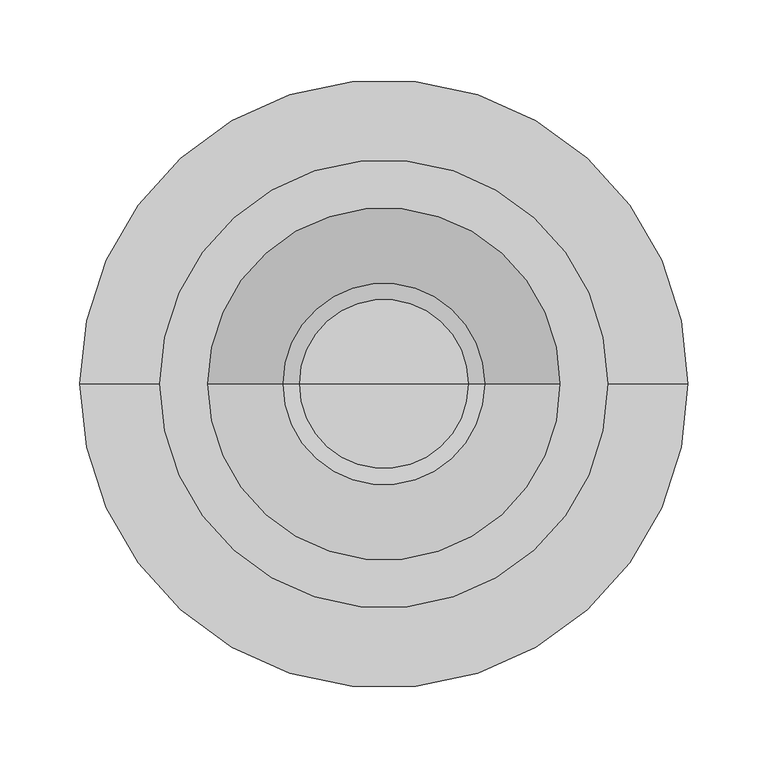
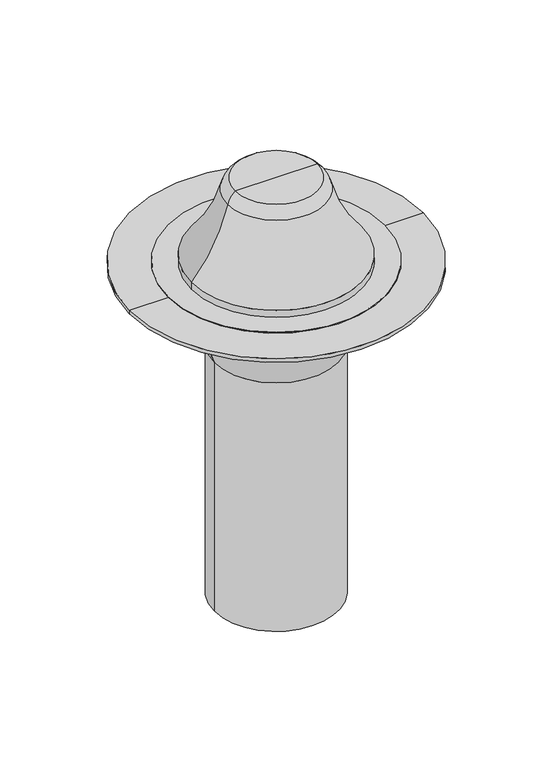
"""IFC4 building model written with IfcOpenShell, lengths in millimetres: proxy geometry, TN_Воронка с обжимным фланцем : Воронка с обжимным закручивающемся фланцем с обогревом Ø160х450мм."""

from ifc_helpers import new_model, si_unit, point, frame, origin, origin_with_axes, origin_2d, place, context, project, spatial, polyline, circle_curve, ellipse_curve, trimmed, segment, composite_curve, outline, extrude, source, transform, mapped, element, save
from ifc_brep_helpers import plane_surface, cylinder_surface, revolved_surface, advanced_brep


def specialty_equipment_53f7e9e1(model_context):
    return source(origin(), model_context, "Body", "SolidModel", [
        advanced_brep(
        [(110.0556416, 0.0, 0.0), (-110.0556416, 0.0, 0.0), (-110.0556416, 0.0, 10.0), (110.0556416, 0.0, 10.0), (0.0, 0.0, 0.0), (52.7728393, 0.0, 115.0), (-52.7728393, 0.0, 115.0), (0.0, 0.0, 115.0), (62.9807579, 0.0, 100.6532382), (-62.9807579, 0.0, 100.6532382)],
        [
            (0, 1, circle_curve(frame((0.0, 0.0, 0.0), z_axis=(0.0, 0.0, 1.0), x_axis=(-1.0, 0.0, 0.0)), 110.0556416)),
            (1, 2),
            (2, 3, circle_curve(frame((0.0, 0.0, 10.0), z_axis=(0.0, 0.0, -1.0), x_axis=(-1.0, 0.0, 0.0)), 110.0556416)),
            (3, 0),
            (1, 0, circle_curve(frame((0.0, 0.0, 0.0), z_axis=(0.0, 0.0, 1.0), x_axis=(-1.0, 0.0, 0.0)), 110.0556416)),
            (3, 2, circle_curve(frame((0.0, 0.0, 10.0), z_axis=(0.0, 0.0, -1.0), x_axis=(-1.0, 0.0, 0.0)), 110.0556416)),
            (4, 1),
            (0, 4),
            (5, 6, circle_curve(frame((0.0, 0.0, 115.0), z_axis=(0.0, 0.0, 1.0), x_axis=(-1.0, 0.0, 0.0)), 52.7728393)),
            (6, 7),
            (7, 5),
            (6, 5, circle_curve(frame((0.0, 0.0, 115.0), z_axis=(0.0, 0.0, 1.0), x_axis=(-1.0, 0.0, 0.0)), 52.7728393)),
            (8, 9, circle_curve(frame((0.0, 0.0, 100.6532382), z_axis=(0.0, 0.0, 1.0), x_axis=(-1.0, 0.0, 0.0)), 62.9807579)),
            (9, 6, circle_curve(frame((-39.8885443, 0.0, 95.0277285), z_axis=(0.0, 1.0, 0.0), x_axis=(1.0, 0.0, 0.0)), 23.7675553)),
            (5, 8, circle_curve(frame((39.8885443, 0.0, 95.0277285), z_axis=(0.0, 1.0, 0.0), x_axis=(-1.0, 0.0, 0.0)), 23.7675553)),
            (9, 8, circle_curve(frame((0.0, 0.0, 100.6532382), z_axis=(0.0, 0.0, 1.0), x_axis=(-1.0, 0.0, 0.0)), 62.9807579)),
            (2, 9, circle_curve(frame((-271.7387744, 0.0, 151.5089197), z_axis=(0.0, -1.0, 0.0), x_axis=(1.0, 0.0, 0.0)), 214.8632351)),
            (8, 3, circle_curve(frame((271.7387744, 0.0, 151.5089197), z_axis=(0.0, -1.0, 0.0), x_axis=(-1.0, 0.0, 0.0)), 214.8632351)),
        ],
        [
            cylinder_surface(frame((0.0, 0.0, 0.0), z_axis=(0.0, 0.0, -1.0), x_axis=(-1.0, 0.0, 0.0)), 110.0556416),
            plane_surface(frame((0.0, 0.0, 0.0), z_axis=(0.0, 0.0, -1.0), x_axis=(-1.0, 0.0, 0.0))),
            plane_surface(frame((0.0, 0.0, 115.0), z_axis=(0.0, 0.0, 1.0), x_axis=(-1.0, 0.0, 0.0))),
            revolved_surface(trimmed(ellipse_curve(frame((-39.8885443, 0.0, 95.0277285), z_axis=(0.0, -1.0, 0.0), x_axis=(1.0, 0.0, 0.0)), 23.7675553, 23.7675553), [point((-52.7728393, 0.0, 115.0))], [point((-62.9807579, 0.0, 100.6532382))], True, "CARTESIAN"), (0.0, 0.0, 0.0), (0.0, 0.0, -1.0)),
            revolved_surface(trimmed(ellipse_curve(frame((-271.7387744, 0.0, 151.5089197), z_axis=(0.0, 1.0, 0.0), x_axis=(1.0, 0.0, 0.0)), 214.8632351, 214.8632351), [point((-62.9807579, 0.0, 100.6532382))], [point((-110.0556416, 0.0, 10.0))], True, "CARTESIAN"), (0.0, 0.0, 0.0), (0.0, 0.0, -1.0)),
        ],
        [
            (0, [[1, 2, 3, 4]]),
            (0, [[5, -4, 6, -2]]),
            (1, [[7, -1, 8]]),
            (1, [[-8, -5, -7]]),
            (2, [[9, 10, 11]]),
            (2, [[12, -11, -10]]),
            (3, [[13, 14, -9, 15]]),
            (3, [[16, -15, -12, -14]]),
            (4, [[-3, 17, -13, 18]]),
            (4, [[-6, -18, -16, -17]]),
        ],
    ),
        extrude(outline(composite_curve([segment(trimmed(circle_curve(origin_2d(), 140.0), [point((-140.0, 0.0))], [point((140.0, 0.0))], False, "CARTESIAN"), True, "CONTINUOUS"), segment(trimmed(circle_curve(origin_2d(), 140.0), [point((140.0, 0.0))], [point((-140.0, 0.0))], False, "CARTESIAN"), True, "CONTINUOUS")], self_intersect=False), holes=[composite_curve([segment(trimmed(circle_curve(origin_2d(), 110.0556416), [point((-110.0556416, 0.0))], [point((110.0556416, 0.0))], True, "CARTESIAN"), True, "CONTINUOUS"), segment(trimmed(circle_curve(origin_2d(), 110.0556416), [point((110.0556416, 0.0))], [point((-110.0556416, 0.0))], True, "CARTESIAN"), True, "CONTINUOUS")], self_intersect=False)]), origin_with_axes(), (0.0, 0.0, 1.0), 1.0),
        advanced_brep(
        [(0.0, 0.0, -450.0), (-80.0, 0.0, -450.0), (80.0, 0.0, -450.0), (190.0, 0.0, 0.0), (-190.0, 0.0, 0.0), (-83.890873, 0.0, 0.0), (83.890873, 0.0, 0.0), (190.0, 0.0, -5.0), (-190.0, 0.0, -5.0), (93.890873, 0.0, -5.0), (-93.890873, 0.0, -5.0), (80.0, 0.0, -110.0), (-80.0, 0.0, -110.0), (-93.890873, 0.0, -71.109127), (93.890873, 0.0, -71.109127), (81.9669914, 0.0, -74.7632135), (-81.9669914, 0.0, -74.7632135), (0.0, 0.0, -74.7632135), (83.890873, 0.0, -69.3768397), (-83.890873, 0.0, -69.3768397)],
        [
            (0, 1),
            (1, 2, circle_curve(frame((0.0, 0.0, -450.0), z_axis=(0.0, 0.0, -1.0), x_axis=(-1.0, 0.0, 0.0)), 80.0)),
            (2, 0),
            (2, 1, circle_curve(frame((0.0, 0.0, -450.0), z_axis=(0.0, 0.0, -1.0), x_axis=(-1.0, 0.0, 0.0)), 80.0)),
            (3, 4, circle_curve(frame((0.0, 0.0, 0.0), z_axis=(0.0, 0.0, 1.0), x_axis=(-1.0, 0.0, 0.0)), 190.0)),
            (4, 5),
            (5, 6, circle_curve(frame((0.0, 0.0, 0.0), z_axis=(0.0, 0.0, -1.0), x_axis=(-1.0, 0.0, 0.0)), 83.890873)),
            (6, 3),
            (4, 3, circle_curve(frame((0.0, 0.0, 0.0), z_axis=(0.0, 0.0, 1.0), x_axis=(-1.0, 0.0, 0.0)), 190.0)),
            (6, 5, circle_curve(frame((0.0, 0.0, 0.0), z_axis=(0.0, 0.0, -1.0), x_axis=(-1.0, 0.0, 0.0)), 83.890873)),
            (7, 8, circle_curve(frame((0.0, 0.0, -5.0), z_axis=(0.0, 0.0, 1.0), x_axis=(-1.0, 0.0, 0.0)), 190.0)),
            (8, 4),
            (3, 7),
            (8, 7, circle_curve(frame((0.0, 0.0, -5.0), z_axis=(0.0, 0.0, 1.0), x_axis=(-1.0, 0.0, 0.0)), 190.0)),
            (9, 10, circle_curve(frame((0.0, 0.0, -5.0), z_axis=(0.0, 0.0, 1.0), x_axis=(-1.0, 0.0, 0.0)), 93.890873)),
            (10, 8),
            (7, 9),
            (10, 9, circle_curve(frame((0.0, 0.0, -5.0), z_axis=(0.0, 0.0, 1.0), x_axis=(-1.0, 0.0, 0.0)), 93.890873)),
            (11, 12, circle_curve(frame((0.0, 0.0, -110.0), z_axis=(0.0, 0.0, 1.0), x_axis=(-1.0, 0.0, 0.0)), 80.0)),
            (12, 13),
            (13, 14, circle_curve(frame((0.0, 0.0, -71.109127), z_axis=(0.0, 0.0, -1.0), x_axis=(-1.0, 0.0, 0.0)), 93.890873)),
            (14, 11),
            (12, 11, circle_curve(frame((0.0, 0.0, -110.0), z_axis=(0.0, 0.0, 1.0), x_axis=(-1.0, 0.0, 0.0)), 80.0)),
            (14, 13, circle_curve(frame((0.0, 0.0, -71.109127), z_axis=(0.0, 0.0, -1.0), x_axis=(-1.0, 0.0, 0.0)), 93.890873)),
            (1, 12),
            (11, 2),
            (15, 16, circle_curve(frame((0.0, 0.0, -74.7632135), z_axis=(0.0, 0.0, 1.0), x_axis=(-1.0, 0.0, 0.0)), 81.9669914)),
            (16, 17),
            (17, 15),
            (16, 15, circle_curve(frame((0.0, 0.0, -74.7632135), z_axis=(0.0, 0.0, 1.0), x_axis=(-1.0, 0.0, 0.0)), 81.9669914)),
            (18, 19, circle_curve(frame((0.0, 0.0, -69.3768397), z_axis=(0.0, 0.0, 1.0), x_axis=(-1.0, 0.0, 0.0)), 83.890873)),
            (19, 16),
            (15, 18),
            (19, 18, circle_curve(frame((0.0, 0.0, -69.3768397), z_axis=(0.0, 0.0, 1.0), x_axis=(-1.0, 0.0, 0.0)), 83.890873)),
            (5, 19),
            (18, 6),
            (13, 10),
            (9, 14),
        ],
        [
            plane_surface(frame((0.0, 0.0, -450.0), z_axis=(0.0, 0.0, -1.0), x_axis=(-1.0, 0.0, 0.0))),
            plane_surface(frame((0.0, 0.0, 0.0), z_axis=(0.0, 0.0, 1.0), x_axis=(-1.0, 0.0, 0.0))),
            cylinder_surface(frame((0.0, 0.0, 0.0), z_axis=(0.0, 0.0, -1.0), x_axis=(-1.0, 0.0, 0.0)), 190.0),
            plane_surface(frame((0.0, 0.0, -5.0), z_axis=(0.0, 0.0, -1.0), x_axis=(-1.0, 0.0, 0.0))),
            revolved_surface(polyline([(-93.890873, 0.0, -71.109127), (-80.0, 0.0, -110.0)]), (0.0, 0.0, 0.0), (0.0, 0.0, -1.0)),
            cylinder_surface(frame((0.0, 0.0, 0.0), z_axis=(0.0, 0.0, -1.0), x_axis=(-1.0, 0.0, 0.0)), 80.0),
            plane_surface(frame((0.0, 0.0, -74.7632135), z_axis=(0.0, 0.0, 1.0), x_axis=(-1.0, 0.0, 0.0))),
            revolved_surface(polyline([(-81.9669914, 0.0, -74.7632135), (-83.890873, 0.0, -69.3768397)]), (0.0, 0.0, 0.0), (0.0, 0.0, -1.0)),
            revolved_surface(polyline([(-83.890873, 0.0, -69.3768397), (-83.890873, 0.0, 0.0)]), (0.0, 0.0, 0.0), (0.0, 0.0, -1.0)),
            cylinder_surface(frame((0.0, 0.0, 0.0), z_axis=(0.0, 0.0, -1.0), x_axis=(-1.0, 0.0, 0.0)), 93.890873),
        ],
        [
            (0, [[1, 2, 3]]),
            (0, [[-3, 4, -1]]),
            (1, [[5, 6, 7, 8]]),
            (1, [[9, -8, 10, -6]]),
            (2, [[11, 12, -5, 13]]),
            (2, [[14, -13, -9, -12]]),
            (3, [[15, 16, -11, 17]]),
            (3, [[18, -17, -14, -16]]),
            (4, [[19, 20, 21, 22]]),
            (4, [[23, -22, 24, -20]]),
            (5, [[-2, 25, -19, 26]]),
            (5, [[-4, -26, -23, -25]]),
            (6, [[27, 28, 29]]),
            (6, [[30, -29, -28]]),
            (7, [[31, 32, -27, 33]]),
            (7, [[34, -33, -30, -32]]),
            (8, [[-7, 35, -31, 36]]),
            (8, [[-10, -36, -34, -35]]),
            (9, [[-21, 37, -15, 38]]),
            (9, [[-24, -38, -18, -37]]),
        ],
    ),
    ])


if __name__ == "__main__":
    model = new_model("IFC4")
    model_context = context("Model", 3, world=origin())
    ifc_project = project(units=[si_unit("LENGTHUNIT", "METRE", prefix="MILLI")], contexts=[model_context])
    site = spatial("IfcSite", under=ifc_project)
    building = spatial("IfcBuilding", under=site)
    placement = place(None, origin())
    specialty_equipment_shape = specialty_equipment_53f7e9e1(model_context)
    element("IfcBuildingElementProxy", 1, Name="TN_Воронка с обжимным фланцем : Воронка с обжимным закручивающемся фланцем с обогревом Ø160х450мм", ObjectType="TN_Воронка с обжимным фланцем : Воронка с обжимным закручивающемся фланцем с обогревом Ø160х450мм", at=placement, inside=building, context=model_context, shape_type="MappedRepresentation", body=[
        mapped(specialty_equipment_shape, transform((0.0, 0.0, 0.0), x_axis=(1.0, 0.0, 0.0), y_axis=(0.0, 1.0, 0.0), z_axis=(0.0, 0.0, 1.0))),
    ])
    save(model, "model.ifc")

# Revit data of these elements
# Type "TN_Воронка с обжимным фланцем : Воронка с обжимным закручивающемся фланцем с обогревом Ø160х450мм"
#   ADSK_Группирование = "Комплектующие и воронки"
#   Description = "Кровельная воронка с обжимным закручивающимся фланцем с обогревом является универсальным средством для отвода воды с поверхности плоских кровель, в устройстве которых использовались ПВХ и ТПО мембраны.\r\n\r\nДля более эффективной работы и удобства монтажа воронка оснащена обжимным закручивающимся фланцем. Благодаря встроенному обогревателю подходит для кровель обогреваемых помещений. Использовать воронку можно во всех климатических регионах, т.к. она не плавится при температуре до +70 С и не становится ломкой до – 55 С.\r\n\r\nДополнительно для защиты от солнца в состав добавлены УФ-стабилизаторы, обеспечивающие устойчивость к ультрафиолетовому и атмосферному воздействию в диапазоне температур от минус 50 до плюс 90 °С.\r\n\r\nБлагодаря механическому способу крепления, воронка подходит для всех типов полимерных кровельных материалов."
#   Manufacturer = "ТехноНИКОЛЬ"
#   URL = "https://shop.tn.ru/voronka-s-obzhimnym-zakruchivajuschemsja-flancem-s-obogrevom-o160h450mm-v3"
#   ADSK_Примечание = ""
#   ADSK_Обозначение = "ТехноНИКОЛЬ"
#   ADSK_Наименование = "Воронка с обжимным закручивающемся фланцем с обогревом Ø160х450мм"
#   ADSK_Масса_Текст = ""
#   ADSK_Марка = ""
#   ADSK_Код изделия = "661130"
#   ADSK_Завод-изготовитель = "ТехноНИКОЛЬ"
#   ADSK_Единица измерения = "шт."
#   ADSK_Группирование = "Комплектующие и воронки"
#   ADSK_URL страницы изделия = "https://shop.tn.ru/voronka-s-obzhimnym-zakruchivajuschemsja-flancem-s-obogrevom-o160h450mm-v3"
#   ADSK_URL документации изделия = "https://shop.tn.ru/media/other_documents/_661125_661124_661134_671701_671702_661132_661131_661130_5.pdf"
#   Тип воронки = 1
#   Радиус = 80 mm
#   Пропускная способность = 11.0 L/s
#   Монтажный диаметр = 160 mm
#   Длина расчетная [instance default] = 450 mm
#   Длина отвода [instance default] = 450 mm
#   ADSK_Масса = 2
#   ADSK_Количество = 1
#   Видимость_Листоуловитель [instance default] = yes
#   Материал_Фланец = TN_Фланец_Красный
#   Материал_Корпус = TN_ПВХ_Черный
#   Default Elevation = 0
# Element 1 (IfcBuildingElementProxy, "TN_Воронка с обжимным фланцем : Воронка с обжимным закручивающемся фланцем с обогревом Ø160х450мм")
#   Materials on its faces: "TN_ПВХ_Черный", "TN_Фланец_Красный"
# Materials
#   "TN_Фланец_Красный": class "Типовые", colour RGB 70 0 0, transparency 0, Cost = 0
#   "TN_ПВХ_Черный": class "Типовые", colour RGB 48 48 48, transparency 0, Cost = 0
